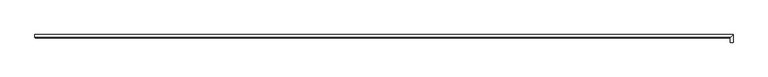
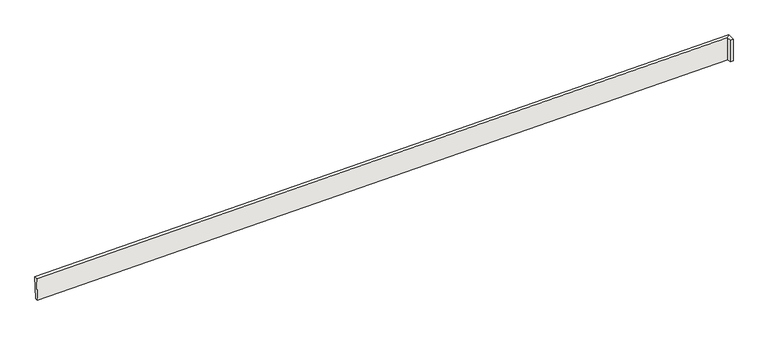
"""IFC4 building model written with IfcOpenShell, lengths in millimetres: slab geometry, FECHAMENTO DECK MADEIRA - RAMPA ENTRADA1 : CC_ND 300 FECHAMENTO 2 x 15 cm DECK MADEIRA - RAMPA ENTRADA."""

from ifc_helpers import new_model, si_unit, origin, place, context, project, spatial, faceted_brep, source, transform, mapped, element, save


def slab_f1ba5172(model_context):
    return source(origin(), model_context, "Body", "Brep", [
        faceted_brep([(-16956.4780242, -1998.3737573, -69.9475924), (-16956.4850119, -2018.3702631, -69.5738214), (-16959.2882946, -2015.5664906, 80.373771), (-16959.281307, -1995.5699847, 80.0), (-12410.281307, -1998.3737573, 15.0439334), (-12430.281307, -2018.3702631, 15.0439334), (-12430.281307, -2015.5664906, 165.0439334), (-12410.281307, -1995.5699847, 165.0439334), (-12410.281307, -2045.5699847, 15.0439334), (-12410.281307, -2045.5699847, 165.0439334), (-12430.281307, -2045.5699847, 165.0439334), (-12430.281307, -2045.5699847, 15.0439334)], [[[0, 1, 2, 3]], [[1, 0, 4, 5]], [[2, 1, 5, 6]], [[3, 2, 6, 7]], [[0, 3, 7, 4]], [[8, 9, 10, 11]], [[5, 4, 8, 11]], [[6, 5, 11, 10]], [[7, 6, 10, 9]], [[4, 7, 9, 8]]]),
    ])


if __name__ == "__main__":
    model = new_model("IFC4")
    model_context = context("Model", 3, world=origin())
    ifc_project = project(units=[si_unit("LENGTHUNIT", "METRE", prefix="MILLI")], contexts=[model_context])
    site = spatial("IfcSite", under=ifc_project)
    building = spatial("IfcBuilding", under=site)
    placement = place(None, origin())
    slab_shape = slab_f1ba5172(model_context)
    element("IfcSlab", 1, ObjectType="FECHAMENTO DECK MADEIRA - RAMPA ENTRADA1 : CC_ND 300 FECHAMENTO 2 x 15 cm DECK MADEIRA - RAMPA ENTRADA", at=placement, inside=building, context=model_context, shape_type="MappedRepresentation", body=[
        mapped(slab_shape, transform((0.0, 0.0, 0.0), x_axis=(1.0, 0.0, 0.0), y_axis=(0.0, 1.0, 0.0), z_axis=(0.0, 0.0, 1.0))),
    ])
    save(model, "model.ifc")

# Revit data of these elements
# Type "FECHAMENTO DECK MADEIRA - RAMPA ENTRADA1 : CC_ND 300 FECHAMENTO 2 x 15 cm DECK MADEIRA - RAMPA ENTRADA"
#   Structural Material = .DECK DE MADEIRA LONGITUDINAL
# Element 1 (IfcSlab, "FECHAMENTO DECK MADEIRA - RAMPA ENTRADA1 : CC_ND 300 FECHAMENTO 2 x 15 cm DECK MADEIRA - RAMPA ENTRADA")
#   Materials on its faces: ".DECK DE MADEIRA LONGITUDINAL"
# Materials
#   ".DECK DE MADEIRA LONGITUDINAL": class ".CC_MADEIRA REVEST.", colour RGB 169 114 85, transparency 0, Description = "Deck de madeira", Cost = 0
